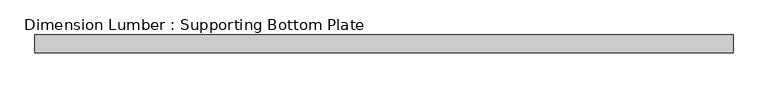
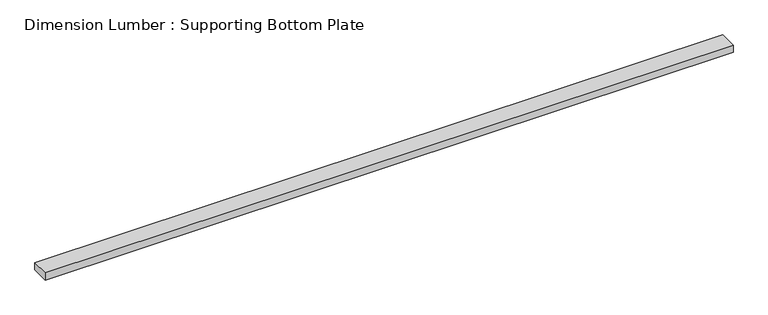
"""IFC4 building model written with IfcOpenShell, lengths in millimetres: beam geometry, Dimension Lumber : Supporting Bottom Plate."""

from ifc_helpers import new_model, si_unit, frame, origin, place, context, project, spatial, polyline, outline, extrude, source, transform, mapped, element, save


def dimension_lumber_supporting_bottom_plate_770482cb(model_context):
    return source(origin(), model_context, "Body", "SweptSolid", [
        extrude(outline(polyline([(1708.546875, 44.45), (1708.546875, -44.45), (-1752.996875, -44.45), (-1752.996875, 44.45), (1708.546875, 44.45)])), frame((0.0, 0.0, -19.05), z_axis=(0.0, 0.0, 1.0), x_axis=(1.0, 0.0, 0.0)), (0.0, 0.0, 1.0), 38.1),
    ])


if __name__ == "__main__":
    model = new_model("IFC4")
    model_context = context("Model", 3, world=origin())
    ifc_project = project(units=[si_unit("LENGTHUNIT", "METRE", prefix="MILLI")], contexts=[model_context])
    site = spatial("IfcSite", under=ifc_project)
    building = spatial("IfcBuilding", under=site)
    placement = place(None, origin())
    dimension_lumber_supporting_bottom_plate_shape = dimension_lumber_supporting_bottom_plate_770482cb(model_context)
    element("IfcBeam", 1, ObjectType="Dimension Lumber : Supporting Bottom Plate", at=placement, inside=building, context=model_context, shape_type="MappedRepresentation", body=[
        mapped(dimension_lumber_supporting_bottom_plate_shape, transform((0.0, 0.0, 0.0), x_axis=(1.0, 0.0, 0.0), y_axis=(0.0, 1.0, 0.0), z_axis=(0.0, 0.0, 1.0))),
    ])
    save(model, "model.ifc")

# Revit data of these elements
# Type "Dimension Lumber : Supporting Bottom Plate"
#   Assembly Code = "B10"
#   A = 0.0364583 SF
#   Length [instance default] = 5' - 0"
#   b = 0' - 3 1/2"
#   d = 0' - 1 1/2"
#   Structural Material [instance default] = Softwood, Lumber
# Element 1 (IfcBeam, "Dimension Lumber : Supporting Bottom Plate")
#   Structural Material = Douglas Fir #2
#   Materials on its faces: "Douglas Fir #2"
# Materials
#   "Softwood, Lumber": class "Wood", colour RGB 223 192 134, transparency 0, Description = "Pinus Echinata", Cost = 0
#   "Douglas Fir #2": class "Wood", colour RGB 223 192 134, transparency 0, Description = "Pinus Echinata", Cost = 0
